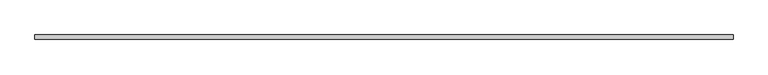
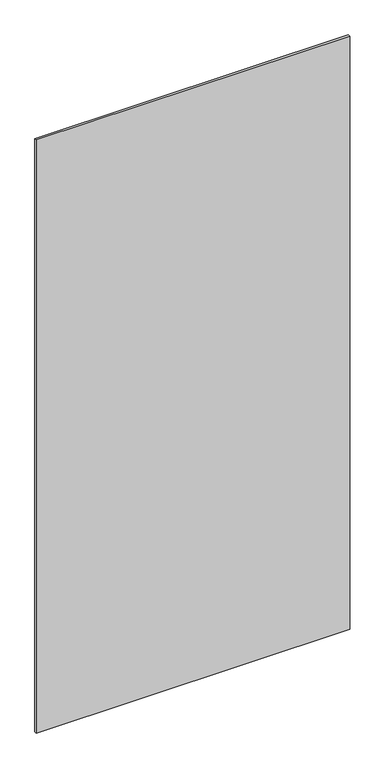
"""IFC4 building model written with IfcOpenShell, lengths in millimetres: proxy geometry, Panel:Panel:300402:Panel:300402 : Panel:Panel:300402:300124:Panel:300402:Panel:300402 : Panel:Panel:300402:300124 : Panel:Panel:300402:Panel:300402 : Panel:Panel:300402:300124:16 : Panel:Panel:300402:Panel:300402 : Panel:Panel:300402:300124:Panel:300402:Panel:300402 : Panel:Panel:300402:300124 : Panel:Panel:300402:Panel:300402 : Panel:Panel:300402:300124:300083."""

from ifc_helpers import new_model, si_unit, frame, origin, place, context, project, spatial, polyline, outline, extrude, source, transform, mapped, element, save


def generic_models_cbda3f88(model_context):
    return source(origin(), model_context, "Body", "SweptSolid", [
        extrude(outline(polyline([(594963.6367239, -579076.8913841), (596182.8367239, -579076.8913841), (596182.8367239, -579084.8288841), (594963.6367239, -579084.8288841), (594963.6367239, -579076.8913841)])), frame((0.0, 0.0, 25.4), z_axis=(0.0, 0.0, 1.0), x_axis=(1.0, 0.0, 0.0)), (0.0, 0.0, 1.0), 2438.4),
    ])


if __name__ == "__main__":
    model = new_model("IFC4")
    model_context = context("Model", 3, world=origin())
    ifc_project = project(units=[si_unit("LENGTHUNIT", "METRE", prefix="MILLI")], contexts=[model_context])
    site = spatial("IfcSite", under=ifc_project)
    building = spatial("IfcBuilding", under=site)
    placement = place(None, origin())
    generic_models_shape = generic_models_cbda3f88(model_context)
    element("IfcBuildingElementProxy", 1, Name="Panel:Panel:300402:Panel:300402 : Panel:Panel:300402:300124:Panel:300402:Panel:300402 : Panel:Panel:300402:300124 : Panel:Panel:300402:Panel:300402 : Panel:Panel:300402:300124:16 : Panel:Panel:300402:Panel:300402 : Panel:Panel:300402:300124:Panel:300402:Panel:300402 : Panel:Panel:300402:300124 : Panel:Panel:300402:Panel:300402 : Panel:Panel:300402:300124:300083", ObjectType="Panel:Panel:300402:Panel:300402 : Panel:Panel:300402:300124:Panel:300402:Panel:300402 : Panel:Panel:300402:300124 : Panel:Panel:300402:Panel:300402 : Panel:Panel:300402:300124:16 : Panel:Panel:300402:Panel:300402 : Panel:Panel:300402:300124:Panel:300402:Panel:300402 : Panel:Panel:300402:300124 : Panel:Panel:300402:Panel:300402 : Panel:Panel:300402:300124:300083", at=placement, inside=building, context=model_context, shape_type="MappedRepresentation", body=[
        mapped(generic_models_shape, transform((0.0, 0.0, 0.0), x_axis=(1.0, 0.0, 0.0), y_axis=(0.0, 1.0, 0.0), z_axis=(0.0, 0.0, 1.0))),
    ])
    save(model, "model.ifc")

# Revit data of these elements
# Type "Panel:Panel:300402:Panel:300402 : Panel:Panel:300402:300124:Panel:300402:Panel:300402 : Panel:Panel:300402:300124 : Panel:Panel:300402:Panel:300402 : Panel:Panel:300402:300124:16 : Panel:Panel:300402:Panel:300402 : Panel:Panel:300402:300124:Panel:300402:Panel:300402 : Panel:Panel:300402:300124 : Panel:Panel:300402:Panel:300402 : Panel:Panel:300402:300124:300083"
#   NameOverride = "Panel:Panel:300402:Panel:300402 : Panel:Panel:300402:300124:Panel:300402:Panel:300402 : Panel:Panel:300402:300124 : Panel:Panel:300402:Panel:300402 : Panel:Panel:300402:300124:300083"
#   ObjectTypeOverride = "Panel:300402:Panel:300402 : Panel:Panel:300402:300124 : Panel:Panel:300402:Panel:300402 : Panel:Panel:300402:300124"
#   Reference = "Panel"
#   Tag = "300083"
# Element 1 (IfcBuildingElementProxy, "Panel:Panel:300402:Panel:300402 : Panel:Panel:300402:300124:Panel:300402:Panel:300402 : Panel:Panel:300402:300124 : Panel:Panel:300402:Panel:300402 : Panel:Panel:300402:300124:16 : Panel:Panel:300402:Panel:300402 : Panel:Panel:300402:300124:Panel:300402:Panel:300402 : Panel:Panel:300402:300124 : Panel:Panel:300402:Panel:300402 : Panel:Panel:300402:300124:300083")
#   Materials on its faces: "5/16\" PHENOLIC RESIN PANELS (CLASS A FLAME SPREAD) - EXPOSED FASTENERS"
# Materials
#   "5/16\" PHENOLIC RESIN PANELS (CLASS A FLAME SPREAD) - EXPOSED FASTENERS": class "Unassigned", colour RGB 64 64 64, transparency 0, Keynote = "M07420000.01", Cost = 0
